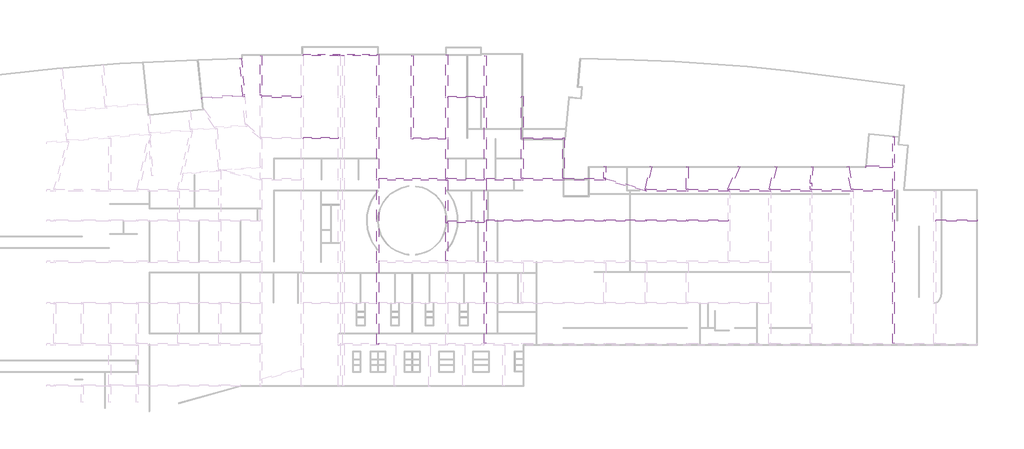
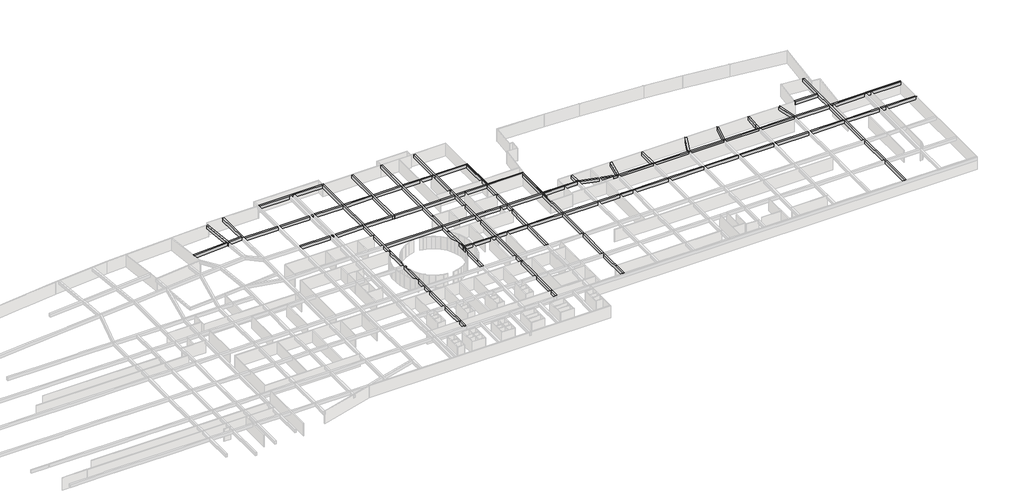
# One storey, part 8 of 8: 36 beams.
"""IFC4 building model written with IfcOpenShell, lengths in millimetres."""

from ifc_helpers import new_model, si_unit, frame, origin, place, context, project, spatial, polyline, outline, extrude, faceted_brep, element, save

model = new_model("IFC4")

# Units and contexts
model_context = context("Model", 3, world=origin())
ifc_project = project(units=[si_unit("LENGTHUNIT", "METRE", prefix="MILLI")], contexts=[model_context])

# Site, building, storey
site = spatial("IfcSite", under=ifc_project)
building = spatial("IfcBuilding", under=site)
storey = spatial("IfcBuildingStorey", under=building, Name="户型图", Elevation=0.0)

# Beams
placement = place(None, origin())
element("IfcBeam", 1, ObjectType="混凝土 - 矩形梁 : KL_beam", at=placement, inside=storey, context=model_context, shape_type="Brep", body=[
    faceted_brep([(535153.8653576, 24850.6327939, 3300.0), (535553.8653576, 24850.6327939, 3300.0), (535553.8653576, 24850.6327939, 2500.0), (535153.8653576, 24850.6327939, 2500.0), (535153.8653576, 18438.6264904, 3300.0), (535153.8653576, 18038.6264904, 3300.0), (535153.8653576, 13338.6264904, 3300.0), (535153.8653576, 12938.6264904, 3300.0), (535153.8653576, 6738.6264904, 3300.0), (535153.8653576, 6338.6264904, 3300.0), (535153.8653576, -2261.3735096, 3300.0), (535153.8653576, -2661.3735096, 3300.0), (535153.8653576, -11261.3735096, 3300.0), (535153.8653576, -11661.3735096, 3300.0), (535153.8653576, -20261.3735096, 3300.0), (535553.8653576, -20261.3735096, 3300.0), (535553.8653576, -11661.3735096, 3300.0), (535553.8653576, -11261.3735096, 3300.0), (535553.8653576, -2661.3735096, 3300.0), (535553.8653576, -2261.3735096, 3300.0), (535553.8653576, 6338.6264904, 3300.0), (535553.8653576, 6738.6264904, 3300.0), (535553.8653576, 12938.6264904, 3300.0), (535553.8653576, 13338.6264904, 3300.0), (535553.8653576, -20261.3735096, 2500.0), (535553.8653576, -11661.3735096, 2500.0), (535553.8653576, -11261.3735096, 2500.0), (535553.8653576, -2661.3735096, 2500.0), (535553.8653576, -2261.3735096, 2500.0), (535553.8653576, 6338.6264904, 2500.0), (535553.8653576, 6738.6264904, 2500.0), (535553.8653576, 12938.6264904, 2500.0), (535553.8653576, 13338.6264904, 2500.0), (535153.8653576, -20261.3735096, 2500.0), (535153.8653576, -11661.3735096, 2500.0), (535153.8653576, -11261.3735096, 2500.0), (535153.8653576, -2661.3735096, 2500.0), (535153.8653576, -2261.3735096, 2500.0), (535153.8653576, 6338.6264904, 2500.0), (535153.8653576, 6738.6264904, 2500.0), (535153.8653576, 12938.6264904, 2500.0), (535153.8653576, 13338.6264904, 2500.0), (535153.8653576, 18038.6264904, 2500.0), (535153.8653576, 18438.6264904, 2500.0)], [[[0, 1, 2, 3]], [[1, 0, 4, 5, 6, 7, 8, 9, 10, 11, 12, 13, 14, 15, 16, 17, 18, 19, 20, 21, 22, 23]], [[2, 1, 23, 22, 21, 20, 19, 18, 17, 16, 15, 24, 25, 26, 27, 28, 29, 30, 31, 32]], [[3, 2, 32, 31, 30, 29, 28, 27, 26, 25, 24, 33, 34, 35, 36, 37, 38, 39, 40, 41, 42, 43]], [[0, 3, 43, 42, 41, 40, 39, 38, 37, 36, 35, 34, 33, 14, 13, 12, 11, 10, 9, 8, 7, 6, 5, 4]], [[15, 14, 33, 24]]]),
])
element("IfcBeam", 2, ObjectType="混凝土 - 矩形梁 : KL_beam", at=placement, inside=storey, context=model_context, shape_type="SweptSolid", body=[
    extrude(outline(polyline([(553653.8653576, 6738.6264904), (553653.8653576, 6338.6264904), (544553.8653576, 6338.6264904), (544553.8653576, 6738.6264904), (553653.8653576, 6738.6264904)])), frame((0.0, 0.0, 2500.0), z_axis=(0.0, 0.0, 1.0), x_axis=(1.0, 0.0, 0.0)), (0.0, 0.0, 1.0), 800.0),
    extrude(outline(polyline([(544153.8653576, 6738.6264904), (544153.8653576, 6338.6264904), (535553.8653576, 6338.6264904), (535553.8653576, 6738.6264904), (544153.8653576, 6738.6264904)])), frame((0.0, 0.0, 2500.0), z_axis=(0.0, 0.0, 1.0), x_axis=(1.0, 0.0, 0.0)), (0.0, 0.0, 1.0), 800.0),
    extrude(outline(polyline([(535153.8653576, 6738.6264904), (535153.8653576, 6338.6264904), (526553.8653576, 6338.6264904), (526553.8653576, 6738.6264904), (535153.8653576, 6738.6264904)])), frame((0.0, 0.0, 2500.0), z_axis=(0.0, 0.0, 1.0), x_axis=(1.0, 0.0, 0.0)), (0.0, 0.0, 1.0), 800.0),
    extrude(outline(polyline([(526153.8653576, 6738.6264904), (526153.8653576, 6338.6264904), (517553.8653576, 6338.6264904), (517553.8653576, 6738.6264904), (526153.8653576, 6738.6264904)])), frame((0.0, 0.0, 2500.0), z_axis=(0.0, 0.0, 1.0), x_axis=(1.0, 0.0, 0.0)), (0.0, 0.0, 1.0), 800.0),
    extrude(outline(polyline([(517153.8653576, 6738.6264904), (517153.8653576, 6338.6264904), (508553.8653576, 6338.6264904), (508553.8653576, 6738.6264904), (517153.8653576, 6738.6264904)])), frame((0.0, 0.0, 2500.0), z_axis=(0.0, 0.0, 1.0), x_axis=(1.0, 0.0, 0.0)), (0.0, 0.0, 1.0), 800.0),
    extrude(outline(polyline([(508153.8653576, 6738.6264904), (508153.8653576, 6338.6264904), (499653.8653576, 6338.6264904), (499653.8653576, 6738.6264904), (508153.8653576, 6738.6264904)])), frame((0.0, 0.0, 2500.0), z_axis=(0.0, 0.0, 1.0), x_axis=(1.0, 0.0, 0.0)), (0.0, 0.0, 1.0), 800.0),
])
element("IfcBeam", 3, ObjectType="混凝土 - 矩形梁 : KL_beam", at=placement, inside=storey, context=model_context, shape_type="Brep", body=[
    faceted_brep([(553518.3052108, 13338.6264904, 3300.0), (553518.3052108, 12938.6264904, 3300.0), (553518.3052108, 12938.6264904, 2500.0), (553518.3052108, 13338.6264904, 2500.0), (535553.8653576, 13338.6264904, 3300.0), (535553.8653576, 12938.6264904, 3300.0), (544153.8653576, 12938.6264904, 3300.0), (544553.8653576, 12938.6264904, 3300.0), (535553.8653576, 12938.6264904, 2500.0), (544153.8653576, 12938.6264904, 2500.0), (544553.8653576, 12938.6264904, 2500.0), (535553.8653576, 13338.6264904, 2500.0)], [[[0, 1, 2, 3]], [[1, 0, 4, 5, 6, 7]], [[2, 1, 7, 6, 5, 8, 9, 10]], [[3, 2, 10, 9, 8, 11]], [[0, 3, 11, 4]], [[5, 4, 11, 8]]]),
    faceted_brep([(535153.8653576, 13338.6264904, 3300.0), (535153.8653576, 12938.6264904, 3300.0), (535153.8653576, 12938.6264904, 2500.0), (535153.8653576, 13338.6264904, 2500.0), (499253.8653576, 13338.6264904, 3300.0), (499253.8653576, 12938.6264904, 3300.0), (499653.8653576, 12938.6264904, 3300.0), (508153.8653576, 12938.6264904, 3300.0), (508553.8653576, 12938.6264904, 3300.0), (517153.8653576, 12938.6264904, 3300.0), (517553.8653576, 12938.6264904, 3300.0), (526153.8653576, 12938.6264904, 3300.0), (526553.8653576, 12938.6264904, 3300.0), (526518.7326348, 13338.6264904, 3300.0), (526111.2459568, 13338.6264904, 3300.0), (517553.8653576, 13338.6264904, 3300.0), (517153.8653576, 13338.6264904, 3300.0), (508609.8536841, 13338.6264904, 3300.0), (508197.6082323, 13338.6264904, 3300.0), (499656.0323963, 13338.6264904, 3300.0), (499253.8653576, 12938.6264904, 2500.0), (499653.8653576, 12938.6264904, 2500.0), (508153.8653576, 12938.6264904, 2500.0), (508553.8653576, 12938.6264904, 2500.0), (517153.8653576, 12938.6264904, 2500.0), (517553.8653576, 12938.6264904, 2500.0), (526153.8653576, 12938.6264904, 2500.0), (526553.8653576, 12938.6264904, 2500.0), (499253.8653576, 13338.6264904, 2500.0), (499656.0323963, 13338.6264904, 2500.0), (508197.6082323, 13338.6264904, 2500.0), (508609.8536841, 13338.6264904, 2500.0), (517153.8653576, 13338.6264904, 2500.0), (517553.8653576, 13338.6264904, 2500.0), (526111.2459568, 13338.6264904, 2500.0), (526518.7326348, 13338.6264904, 2500.0)], [[[0, 1, 2, 3]], [[4, 5, 6, 7, 8, 9, 10, 11, 12, 1, 0, 13, 14, 15, 16, 17, 18, 19]], [[5, 20, 21, 22, 23, 24, 25, 26, 27, 2, 1, 12, 11, 10, 9, 8, 7, 6]], [[20, 28, 29, 30, 31, 32, 33, 34, 35, 3, 2, 27, 26, 25, 24, 23, 22, 21]], [[28, 4, 19, 18, 17, 16, 15, 14, 13, 0, 3, 35, 34, 33, 32, 31, 30, 29]], [[5, 4, 28, 20]]]),
])
element("IfcBeam", 4, ObjectType="混凝土 - 矩形梁 : KL_beam", at=placement, inside=storey, context=model_context, shape_type="Brep", body=[
    faceted_brep([(499253.8653576, 6338.6264904, 3300.0), (499253.8653576, 6738.6264904, 3300.0), (490553.8653576, 6738.6264904, 3300.0), (490153.8653576, 6738.6264904, 3300.0), (481553.8653576, 6738.6264904, 3300.0), (481153.8653576, 6738.6264904, 3300.0), (472553.8653576, 6738.6264904, 3300.0), (472153.8653576, 6738.6264904, 3300.0), (463553.8653576, 6738.6264904, 3300.0), (463153.8653576, 6738.6264904, 3300.0), (454553.8653576, 6738.6264904, 3300.0), (454153.8653576, 6738.6264904, 3300.0), (446453.8653576, 6738.6264904, 3300.0), (446453.8653576, 6338.6264904, 3300.0), (454153.8653576, 6338.6264904, 3300.0), (454553.8653576, 6338.6264904, 3300.0), (463153.8653576, 6338.6264904, 3300.0), (463553.8653576, 6338.6264904, 3300.0), (472153.8653576, 6338.6264904, 3300.0), (472553.8653576, 6338.6264904, 3300.0), (481153.8653576, 6338.6264904, 3300.0), (481553.8653576, 6338.6264904, 3300.0), (490153.8653576, 6338.6264904, 3300.0), (490553.8653576, 6338.6264904, 3300.0), (499253.8653576, 6338.6264904, 2500.0), (446453.8653576, 6338.6264904, 2500.0), (454153.8653576, 6338.6264904, 2500.0), (454553.8653576, 6338.6264904, 2500.0), (463153.8653576, 6338.6264904, 2500.0), (463553.8653576, 6338.6264904, 2500.0), (472153.8653576, 6338.6264904, 2500.0), (472553.8653576, 6338.6264904, 2500.0), (481153.8653576, 6338.6264904, 2500.0), (481553.8653576, 6338.6264904, 2500.0), (490153.8653576, 6338.6264904, 2500.0), (490553.8653576, 6338.6264904, 2500.0), (499253.8653576, 6738.6264904, 2500.0), (446453.8653576, 6738.6264904, 2500.0), (454153.8653576, 6738.6264904, 2500.0), (454553.8653576, 6738.6264904, 2500.0), (463153.8653576, 6738.6264904, 2500.0), (463553.8653576, 6738.6264904, 2500.0), (472153.8653576, 6738.6264904, 2500.0), (472553.8653576, 6738.6264904, 2500.0), (481153.8653576, 6738.6264904, 2500.0), (481553.8653576, 6738.6264904, 2500.0), (490153.8653576, 6738.6264904, 2500.0), (490553.8653576, 6738.6264904, 2500.0)], [[[0, 1, 2, 3, 4, 5, 6, 7, 8, 9, 10, 11, 12, 13, 14, 15, 16, 17, 18, 19, 20, 21, 22, 23]], [[24, 0, 23, 22, 21, 20, 19, 18, 17, 16, 15, 14, 13, 25, 26, 27, 28, 29, 30, 31, 32, 33, 34, 35]], [[36, 24, 35, 34, 33, 32, 31, 30, 29, 28, 27, 26, 25, 37, 38, 39, 40, 41, 42, 43, 44, 45, 46, 47]], [[1, 36, 47, 46, 45, 44, 43, 42, 41, 40, 39, 38, 37, 12, 11, 10, 9, 8, 7, 6, 5, 4, 3, 2]], [[1, 0, 24, 36]], [[13, 12, 37, 25]]]),
])
element("IfcBeam", 5, ObjectType="混凝土 - 矩形梁 : KL_beam", at=placement, inside=storey, context=model_context, shape_type="Brep", body=[
    faceted_brep([(481153.8653576, 13338.6264904, 3300.0), (481153.8653576, 13157.8287437, 3300.0), (481153.8653576, 12984.9708278, 3300.0), (481153.8653576, 12938.6264904, 3300.0), (481553.8653576, 12938.6264904, 3300.0), (490153.8653576, 12938.6264904, 3300.0), (490553.8653576, 12938.6264904, 3300.0), (499253.8653576, 12938.6264904, 3300.0), (499253.8653576, 13338.6264904, 3300.0), (499221.4882454, 13338.6264904, 3300.0), (490553.8653576, 13338.6264904, 3300.0), (490153.8653576, 13338.6264904, 3300.0), (481596.3487482, 13338.6264904, 3300.0), (481188.9056055, 13338.6264904, 3300.0), (481153.8653576, 13338.6264904, 2500.0), (499253.8653576, 13338.6264904, 2500.0), (499221.4882454, 13338.6264904, 2500.0), (490553.8653576, 13338.6264904, 2500.0), (490153.8653576, 13338.6264904, 2500.0), (481596.3487482, 13338.6264904, 2500.0), (481188.9056055, 13338.6264904, 2500.0), (481153.8653576, 12938.6264904, 2500.0), (481153.8653576, 12984.9708278, 2500.0), (481153.8653576, 13157.8287437, 2500.0), (499253.8653576, 12938.6264904, 2500.0), (490553.8653576, 12938.6264904, 2500.0), (490153.8653576, 12938.6264904, 2500.0), (481553.8653576, 12938.6264904, 2500.0)], [[[0, 1, 2, 3, 4, 5, 6, 7, 8, 9, 10, 11, 12, 13]], [[14, 0, 13, 12, 11, 10, 9, 8, 15, 16, 17, 18, 19, 20]], [[21, 22, 23, 14, 20, 19, 18, 17, 16, 15, 24, 25, 26, 27]], [[3, 21, 27, 26, 25, 24, 7, 6, 5, 4]], [[3, 2, 1, 0, 14, 23, 22, 21]], [[8, 7, 24, 15]]]),
])
element("IfcBeam", 6, ObjectType="混凝土 - 矩形梁 : KL_beam", at=placement, inside=storey, context=model_context, shape_type="Brep", body=[
    faceted_brep([(472553.8653576, 15338.6264904, 3300.0), (472553.8653576, 15692.282153, 3300.0), (472553.8653576, 15738.6264904, 3300.0), (472380.0740924, 15738.6264904, 3300.0), (472153.8653576, 15738.6264904, 3300.0), (463553.8653576, 15738.6264904, 3300.0), (463153.8653576, 15738.6264904, 3300.0), (454553.8653576, 15738.6264904, 3300.0), (454153.8653576, 15738.6264904, 3300.0), (446453.8653576, 15738.6264904, 3300.0), (446453.8653576, 15338.6264904, 3300.0), (454153.8653576, 15338.6264904, 3300.0), (454553.8653576, 15338.6264904, 3300.0), (463153.8653576, 15338.6264904, 3300.0), (463553.8653576, 15338.6264904, 3300.0), (472153.8653576, 15338.6264904, 3300.0), (472553.8653576, 15738.6264904, 2500.0), (472380.0740924, 15738.6264904, 2500.0), (472153.8653576, 15738.6264904, 2500.0), (463553.8653576, 15738.6264904, 2500.0), (463153.8653576, 15738.6264904, 2500.0), (454553.8653576, 15738.6264904, 2500.0), (454153.8653576, 15738.6264904, 2500.0), (446453.8653576, 15738.6264904, 2500.0), (472553.8653576, 15692.282153, 2500.0), (472553.8653576, 15338.6264904, 2500.0), (472153.8653576, 15338.6264904, 2500.0), (463553.8653576, 15338.6264904, 2500.0), (463153.8653576, 15338.6264904, 2500.0), (454553.8653576, 15338.6264904, 2500.0), (454153.8653576, 15338.6264904, 2500.0), (446453.8653576, 15338.6264904, 2500.0)], [[[0, 1, 2, 3, 4, 5, 6, 7, 8, 9, 10, 11, 12, 13, 14, 15]], [[2, 16, 17, 18, 19, 20, 21, 22, 23, 9, 8, 7, 6, 5, 4, 3]], [[16, 24, 25, 26, 27, 28, 29, 30, 31, 23, 22, 21, 20, 19, 18, 17]], [[25, 0, 15, 14, 13, 12, 11, 10, 31, 30, 29, 28, 27, 26]], [[2, 1, 0, 25, 24, 16]], [[10, 9, 23, 31]]]),
])
element("IfcBeam", 7, ObjectType="混凝土 - 矩形梁 : KL_beam", at=placement, inside=storey, context=model_context, shape_type="Brep", body=[
    faceted_brep([(463153.8653576, -20261.3735096, 3300.0), (463553.8653576, -20261.3735096, 3300.0), (463553.8653576, -11661.3735096, 3300.0), (463153.8653576, -11661.3735096, 3300.0), (463553.8653576, -20261.3735096, 2500.0), (463553.8653576, -11661.3735096, 2500.0), (463153.8653576, -20261.3735096, 2500.0), (463153.8653576, -11661.3735096, 2500.0)], [[[0, 1, 2, 3]], [[1, 4, 5, 2]], [[4, 6, 7, 5]], [[6, 0, 3, 7]], [[1, 0, 6, 4]], [[3, 2, 5, 7]]]),
    faceted_brep([(463553.8653576, -2261.3735096, 3300.0), (463153.8653576, -2261.3735096, 3300.0), (463153.8653576, -2261.3735096, 2500.0), (463553.8653576, -2261.3735096, 2500.0), (463153.8653576, 6338.6264904, 3300.0), (463553.8653576, 6338.6264904, 3300.0), (463553.8653576, 6338.6264904, 2500.0), (463153.8653576, 6338.6264904, 2500.0)], [[[0, 1, 2, 3]], [[4, 5, 6, 7]], [[1, 0, 5, 4]], [[0, 3, 6, 5]], [[3, 2, 7, 6]], [[2, 1, 4, 7]]]),
    faceted_brep([(463153.8653576, -2661.3735096, 3300.0), (463553.8653576, -2661.3735096, 3300.0), (463553.8653576, -2661.3735096, 2500.0), (463153.8653576, -2661.3735096, 2500.0), (463553.8653576, -11261.3735096, 3300.0), (463153.8653576, -11261.3735096, 3300.0), (463153.8653576, -11261.3735096, 2500.0), (463553.8653576, -11261.3735096, 2500.0)], [[[0, 1, 2, 3]], [[4, 5, 6, 7]], [[1, 0, 5, 4]], [[2, 1, 4, 7]], [[3, 2, 7, 6]], [[0, 3, 6, 5]]]),
    faceted_brep([(463153.8653576, 6738.6264904, 3300.0), (463553.8653576, 6738.6264904, 3300.0), (463553.8653576, 15338.6264904, 3300.0), (463153.8653576, 15338.6264904, 3300.0), (463553.8653576, 6738.6264904, 2500.0), (463553.8653576, 15338.6264904, 2500.0), (463153.8653576, 6738.6264904, 2500.0), (463153.8653576, 15338.6264904, 2500.0)], [[[0, 1, 2, 3]], [[1, 4, 5, 2]], [[4, 6, 7, 5]], [[6, 0, 3, 7]], [[1, 0, 6, 4]], [[3, 2, 5, 7]]]),
    faceted_brep([(463553.8653576, 15738.6264904, 3300.0), (463153.8653576, 15738.6264904, 3300.0), (463153.8653576, 15738.6264904, 2500.0), (463553.8653576, 15738.6264904, 2500.0), (463153.8653576, 24638.6264904, 3300.0), (463553.8653576, 24638.6264904, 3300.0), (463553.8653576, 24638.6264904, 2500.0), (463153.8653576, 24638.6264904, 2500.0), (463153.8653576, 24238.6264904, 3300.0), (463153.8653576, 24238.6264904, 2500.0)], [[[0, 1, 2, 3]], [[4, 5, 6, 7]], [[5, 4, 8, 1, 0]], [[6, 5, 0, 3]], [[7, 6, 3, 2, 9]], [[4, 7, 9, 2, 1, 8]]]),
])
element("IfcBeam", 8, ObjectType="混凝土 - 矩形梁 : KL_beam", at=placement, inside=storey, context=model_context, shape_type="SweptSolid", body=[
    extrude(outline(polyline([(517153.8653576, 14643.8636747), (517553.8653576, 14633.3893061), (517553.8653576, 13338.6264904), (517153.8653576, 13338.6264904), (517153.8653576, 14643.8636747)])), frame((0.0, 0.0, 2500.0), z_axis=(0.0, 0.0, 1.0), x_axis=(1.0, 0.0, 0.0)), (0.0, 0.0, 1.0), 800.0),
])
element("IfcBeam", 9, ObjectType="混凝土 - 矩形梁 : KL_beam", at=placement, inside=storey, context=model_context, shape_type="SweptSolid", body=[
    extrude(outline(polyline([(517342.7828465, 18248.6241033), (517742.2346604, 18227.6897208), (517553.8653576, 14633.3893061), (517153.8653576, 14643.8636747), (517342.7828465, 18248.6241033)])), frame((0.0, 0.0, 2500.0), z_axis=(0.0, 0.0, 1.0), x_axis=(1.0, 0.0, 0.0)), (0.0, 0.0, 1.0), 800.0),
])
element("IfcBeam", 10, ObjectType="混凝土 - 矩形梁 : KL_beam", at=placement, inside=storey, context=model_context, shape_type="SweptSolid", body=[
    extrude(outline(polyline([(525146.7934929, 18300.3042867), (525539.4443663, 18376.6278849), (526518.7326348, 13338.6264904), (526111.2459568, 13338.6264904), (525146.7934929, 18300.3042867)])), frame((0.0, 0.0, 2500.0), z_axis=(0.0, 0.0, 1.0), x_axis=(1.0, 0.0, 0.0)), (0.0, 0.0, 1.0), 800.0),
])
element("IfcBeam", 11, ObjectType="混凝土 - 矩形梁 : KL_beam", at=placement, inside=storey, context=model_context, shape_type="SweptSolid", body=[
    extrude(outline(polyline([(529331.7779591, 18038.6264904), (529331.7779591, 18438.6264904), (535153.8653576, 18438.6264904), (535153.8653576, 18038.6264904), (529331.7779591, 18038.6264904)])), frame((0.0, 0.0, 2500.0), z_axis=(0.0, 0.0, 1.0), x_axis=(1.0, 0.0, 0.0)), (0.0, 0.0, 1.0), 800.0),
])
element("IfcBeam", 12, ObjectType="混凝土 - 矩形梁 : KL_beam", at=placement, inside=storey, context=model_context, shape_type="SweptSolid", body=[
    extrude(outline(polyline([(509441.992259, 18329.5782188), (509830.1105496, 18232.8094606), (508609.8536841, 13338.6264904), (508197.6082323, 13338.6264904), (509441.992259, 18329.5782188)])), frame((0.0, 0.0, 2500.0), z_axis=(0.0, 0.0, 1.0), x_axis=(1.0, 0.0, 0.0)), (0.0, 0.0, 1.0), 800.0),
])
element("IfcBeam", 13, ObjectType="混凝土 - 矩形梁 : KL_beam", at=placement, inside=storey, context=model_context, shape_type="Brep", body=[
    faceted_brep([(501377.0189815, 18416.7386747, 3300.0), (501745.2209229, 18260.4462233, 3300.0), (501745.2209229, 18260.4462233, 2500.0), (501377.0189815, 18416.7386747, 2500.0), (499221.4882454, 13338.6264904, 3300.0), (499253.8653576, 13338.6264904, 3300.0), (499656.0323963, 13338.6264904, 3300.0), (499656.0323963, 13338.6264904, 2500.0), (499253.8653576, 13338.6264904, 2500.0), (499221.4882454, 13338.6264904, 2500.0)], [[[0, 1, 2, 3]], [[1, 0, 4, 5, 6]], [[2, 1, 6, 7]], [[3, 2, 7, 8, 9]], [[0, 3, 9, 4]], [[4, 9, 8, 7, 6, 5]]]),
])
element("IfcBeam", 14, ObjectType="混凝土 - 矩形梁 : KL_beam", at=placement, inside=storey, context=model_context, shape_type="SweptSolid", body=[
    extrude(outline(polyline([(490153.8653576, 18238.6264904), (490553.8653576, 18238.6264904), (490553.8653576, 13338.6264904), (490153.8653576, 13338.6264904), (490153.8653576, 18238.6264904)])), frame((0.0, 0.0, 2500.0), z_axis=(0.0, 0.0, 1.0), x_axis=(1.0, 0.0, 0.0)), (0.0, 0.0, 1.0), 800.0),
])
element("IfcBeam", 15, ObjectType="混凝土 - 矩形梁 : KL_beam", at=placement, inside=storey, context=model_context, shape_type="Brep", body=[
    faceted_brep([(482165.253861, 18376.3067336, 3300.0), (482557.9466891, 18300.1992914, 3300.0), (482557.9466891, 18300.1992914, 2500.0), (482165.253861, 18376.3067336, 2500.0), (481198.3001251, 13387.0995484, 3300.0), (481188.9056055, 13338.6264904, 3300.0), (481553.8653576, 13338.6264904, 3300.0), (481596.3487482, 13338.6264904, 3300.0), (481596.3487482, 13338.6264904, 2500.0), (481553.8653576, 13338.6264904, 2500.0), (481188.9056055, 13338.6264904, 2500.0), (481198.3001251, 13387.0995484, 2500.0)], [[[0, 1, 2, 3]], [[1, 0, 4, 5, 6, 7]], [[2, 1, 7, 8]], [[3, 2, 8, 9, 10, 11]], [[0, 3, 11, 10, 5, 4]], [[8, 7, 6, 5, 10, 9]]]),
    faceted_brep([(481153.8653576, 13157.8287437, 3300.0), (481153.8653576, 12984.9708278, 3300.0), (481153.8653576, 12984.9708278, 2500.0), (481153.8653576, 13157.8287437, 2500.0), (481122.0102694, 12993.465518, 3300.0), (481122.0102694, 12993.465518, 2500.0)], [[[0, 1, 2, 3]], [[4, 5, 2, 1]], [[1, 0, 4]], [[3, 2, 5]], [[0, 3, 5, 4]]]),
])
element("IfcBeam", 16, ObjectType="混凝土 - 矩形梁 : KL_beam", at=placement, inside=storey, context=model_context, shape_type="Brep", body=[
    faceted_brep([(481198.3001251, 13387.0995484, 3300.0), (481198.3001251, 13387.0995484, 2500.0), (472553.8653576, 15692.282153, 2500.0), (472553.8653576, 15692.282153, 3300.0), (481153.8653576, 13338.6264904, 3300.0), (481153.8653576, 13338.6264904, 2500.0), (481188.9056055, 13338.6264904, 2500.0), (481188.9056055, 13338.6264904, 3300.0), (481153.8653576, 13157.8287437, 3300.0), (481153.8653576, 13157.8287437, 2500.0), (472553.8653576, 15338.6264904, 3300.0), (472553.8653576, 15278.3041611, 3300.0), (481122.0102694, 12993.465518, 3300.0), (481122.0102694, 12993.465518, 2500.0), (472553.8653576, 15278.3041611, 2500.0), (472553.8653576, 15338.6264904, 2500.0)], [[[0, 1, 2, 3]], [[4, 5, 6, 7]], [[5, 4, 8, 9]], [[8, 4, 7, 0, 3, 10, 11, 12]], [[13, 12, 11, 14]], [[6, 5, 9, 13, 14, 15, 2, 1]], [[1, 0, 7, 6]], [[9, 8, 12, 13]], [[3, 2, 15, 14, 11, 10]]]),
    faceted_brep([(472153.8653576, 15738.6264904, 2500.0), (472153.8653576, 15738.6264904, 3300.0), (472153.8653576, 15798.9488197, 3300.0), (472153.8653576, 15798.9488197, 2500.0), (472380.0740924, 15738.6264904, 2500.0), (472380.0740924, 15738.6264904, 3300.0)], [[[0, 1, 2, 3]], [[4, 5, 1, 0]], [[4, 3, 2, 5]], [[5, 2, 1]], [[3, 4, 0]]]),
])
element("IfcBeam", 17, ObjectType="混凝土 - 矩形梁 : KL_beam", at=placement, inside=storey, context=model_context, shape_type="SweptSolid", body=[
    extrude(outline(polyline([(472153.8653576, 18338.6264904), (472553.8653576, 18338.6264904), (472553.8653576, 15738.6264904), (472380.0740924, 15738.6264904), (472153.8653576, 15798.9488197), (472153.8653576, 18338.6264904)])), frame((0.0, 0.0, 2500.0), z_axis=(0.0, 0.0, 1.0), x_axis=(1.0, 0.0, 0.0)), (0.0, 0.0, 1.0), 800.0),
])
element("IfcBeam", 18, ObjectType="混凝土 - 矩形梁 : KL_beam", at=placement, inside=storey, context=model_context, shape_type="Brep", body=[
    faceted_brep([(454153.8653576, -2261.3735096, 3300.0), (454553.8653576, -2261.3735096, 3300.0), (454553.8653576, 6338.6264904, 3300.0), (454153.8653576, 6338.6264904, 3300.0), (454553.8653576, -2261.3735096, 2500.0), (454553.8653576, 6338.6264904, 2500.0), (454153.8653576, -2261.3735096, 2500.0), (454153.8653576, 6338.6264904, 2500.0)], [[[0, 1, 2, 3]], [[1, 4, 5, 2]], [[4, 6, 7, 5]], [[6, 0, 3, 7]], [[1, 0, 6, 4]], [[3, 2, 5, 7]]]),
    faceted_brep([(454553.8653576, 6738.6264904, 3300.0), (454153.8653576, 6738.6264904, 3300.0), (454153.8653576, 6738.6264904, 2500.0), (454553.8653576, 6738.6264904, 2500.0), (454153.8653576, 15338.6264904, 3300.0), (454553.8653576, 15338.6264904, 3300.0), (454553.8653576, 15338.6264904, 2500.0), (454153.8653576, 15338.6264904, 2500.0)], [[[0, 1, 2, 3]], [[4, 5, 6, 7]], [[1, 0, 5, 4]], [[0, 3, 6, 5]], [[3, 2, 7, 6]], [[2, 1, 4, 7]]]),
    faceted_brep([(454553.8653576, 33688.6264755, 3300.0), (454153.8653576, 33688.6264755, 3300.0), (454153.8653576, 33288.6264755, 3300.0), (454153.8653576, 24638.6264904, 3300.0), (454153.8653576, 24238.6264904, 3300.0), (454153.8653576, 15738.6264904, 3300.0), (454553.8653576, 15738.6264904, 3300.0), (454553.8653576, 24238.6264904, 3300.0), (454553.8653576, 24638.6264904, 3300.0), (454553.8653576, 33688.6264755, 2500.0), (454553.8653576, 15738.6264904, 2500.0), (454553.8653576, 24238.6264904, 2500.0), (454553.8653576, 24638.6264904, 2500.0), (454153.8653576, 33688.6264755, 2500.0), (454153.8653576, 15738.6264904, 2500.0), (454153.8653576, 24238.6264904, 2500.0), (454153.8653576, 24638.6264904, 2500.0), (454153.8653576, 33288.6264755, 2500.0)], [[[0, 1, 2, 3, 4, 5, 6, 7, 8]], [[9, 0, 8, 7, 6, 10, 11, 12]], [[13, 9, 12, 11, 10, 14, 15, 16, 17]], [[1, 13, 17, 16, 15, 14, 5, 4, 3, 2]], [[6, 5, 14, 10]], [[1, 0, 9, 13]]]),
])
element("IfcBeam", 19, ObjectType="混凝土 - 矩形梁 : KL_beam", at=placement, inside=storey, context=model_context, shape_type="Brep", body=[
    faceted_brep([(446453.8653576, 42538.6264904, 3300.0), (446453.8653576, 42538.6264904, 2500.0), (446053.8653576, 42538.6264904, 2500.0), (446053.8653576, 42538.6264904, 3300.0), (446053.8653576, 33688.6264755, 3300.0), (446053.8653576, 33288.6264755, 3300.0), (446053.8653576, 24638.6264904, 3300.0), (446053.8653576, 24238.6264904, 3300.0), (446053.8653576, 15738.6264904, 3300.0), (446053.8653576, 15338.6264904, 3300.0), (446053.8653576, 6488.6264674, 3300.0), (446053.8653576, 6088.6264674, 3300.0), (446053.8653576, -2261.3735096, 3300.0), (446053.8653576, -2661.3735096, 3300.0), (446053.8653576, -11261.3735096, 3300.0), (446053.8653576, -11661.3735096, 3300.0), (446053.8653576, -20261.3735096, 3300.0), (446453.8653576, -20261.3735096, 3300.0), (446453.8653576, -11661.3735096, 3300.0), (446453.8653576, -11261.3735096, 3300.0), (446453.8653576, -2661.3735096, 3300.0), (446453.8653576, -2261.3735096, 3300.0), (446453.8653576, 6338.6264904, 3300.0), (446453.8653576, 6738.6264904, 3300.0), (446453.8653576, 15338.6264904, 3300.0), (446453.8653576, 15738.6264904, 3300.0), (446453.8653576, 24238.6264904, 3300.0), (446453.8653576, 24638.6264904, 3300.0), (446453.8653576, 33288.6264755, 3300.0), (446453.8653576, 33688.6264755, 3300.0), (446053.8653576, 33688.6264755, 2500.0), (446053.8653576, 33288.6264755, 2500.0), (446053.8653576, 24638.6264904, 2500.0), (446053.8653576, 24238.6264904, 2500.0), (446053.8653576, 15738.6264904, 2500.0), (446053.8653576, 15338.6264904, 2500.0), (446053.8653576, 6488.6264674, 2500.0), (446053.8653576, 6088.6264674, 2500.0), (446053.8653576, -2261.3735096, 2500.0), (446053.8653576, -2661.3735096, 2500.0), (446053.8653576, -11261.3735096, 2500.0), (446053.8653576, -11661.3735096, 2500.0), (446053.8653576, -20261.3735096, 2500.0), (446453.8653576, 33688.6264755, 2500.0), (446453.8653576, 33288.6264755, 2500.0), (446453.8653576, 24638.6264904, 2500.0), (446453.8653576, 24238.6264904, 2500.0), (446453.8653576, 15738.6264904, 2500.0), (446453.8653576, 15338.6264904, 2500.0), (446453.8653576, 6738.6264904, 2500.0), (446453.8653576, 6338.6264904, 2500.0), (446453.8653576, -2261.3735096, 2500.0), (446453.8653576, -2661.3735096, 2500.0), (446453.8653576, -11261.3735096, 2500.0), (446453.8653576, -11661.3735096, 2500.0), (446453.8653576, -20261.3735096, 2500.0)], [[[0, 1, 2, 3]], [[0, 3, 4, 5, 6, 7, 8, 9, 10, 11, 12, 13, 14, 15, 16, 17, 18, 19, 20, 21, 22, 23, 24, 25, 26, 27, 28, 29]], [[3, 2, 30, 31, 32, 33, 34, 35, 36, 37, 38, 39, 40, 41, 42, 16, 15, 14, 13, 12, 11, 10, 9, 8, 7, 6, 5, 4]], [[2, 1, 43, 44, 45, 46, 47, 48, 49, 50, 51, 52, 53, 54, 55, 42, 41, 40, 39, 38, 37, 36, 35, 34, 33, 32, 31, 30]], [[1, 0, 29, 28, 27, 26, 25, 24, 23, 22, 21, 20, 19, 18, 17, 55, 54, 53, 52, 51, 50, 49, 48, 47, 46, 45, 44, 43]], [[17, 16, 42, 55]]]),
])
element("IfcBeam", 20, ObjectType="混凝土 - 矩形梁 : KL_beam", at=placement, inside=storey, context=model_context, shape_type="Brep", body=[
    faceted_brep([(437653.8653576, 15738.6264904, 3300.0), (437653.8653576, 15338.6264904, 3300.0), (438053.8653576, 15338.6264904, 3300.0), (446053.8653576, 15338.6264904, 3300.0), (446053.8653576, 15738.6264904, 3300.0), (438053.8653576, 15738.6264904, 3300.0), (437653.8653576, 15738.6264904, 2500.0), (446053.8653576, 15738.6264904, 2500.0), (438053.8653576, 15738.6264904, 2500.0), (437653.8653576, 15338.6264904, 2500.0), (446053.8653576, 15338.6264904, 2500.0), (438053.8653576, 15338.6264904, 2500.0)], [[[0, 1, 2, 3, 4, 5]], [[6, 0, 5, 4, 7, 8]], [[9, 6, 8, 7, 10, 11]], [[1, 9, 11, 10, 3, 2]], [[4, 3, 10, 7]], [[1, 0, 6, 9]]]),
])
element("IfcBeam", 21, ObjectType="混凝土 - 矩形梁 : KL_beam", at=placement, inside=storey, context=model_context, shape_type="Brep", body=[
    faceted_brep([(437653.8653576, 42735.0986184, 3300.0), (438053.8653576, 42735.0986184, 3300.0), (438053.8653576, 42735.0986184, 2500.0), (437653.8653576, 42735.0986184, 2500.0), (437653.8653576, 33688.6264755, 3300.0), (437653.8653576, 33288.6264755, 3300.0), (437653.8653576, 24638.6264904, 3300.0), (437653.8653576, 24238.6264904, 3300.0), (437653.8653576, 15738.6264904, 3300.0), (438053.8653576, 15738.6264904, 3300.0), (438053.8653576, 24238.6264904, 3300.0), (438053.8653576, 24638.6264904, 3300.0), (438053.8653576, 33288.6264755, 3300.0), (438053.8653576, 33688.6264755, 3300.0), (438053.8653576, 15738.6264904, 2500.0), (438053.8653576, 24238.6264904, 2500.0), (438053.8653576, 24638.6264904, 2500.0), (438053.8653576, 33288.6264755, 2500.0), (438053.8653576, 33688.6264755, 2500.0), (437653.8653576, 15738.6264904, 2500.0), (437653.8653576, 24238.6264904, 2500.0), (437653.8653576, 24638.6264904, 2500.0), (437653.8653576, 33288.6264755, 2500.0), (437653.8653576, 33688.6264755, 2500.0)], [[[0, 1, 2, 3]], [[1, 0, 4, 5, 6, 7, 8, 9, 10, 11, 12, 13]], [[2, 1, 13, 12, 11, 10, 9, 14, 15, 16, 17, 18]], [[3, 2, 18, 17, 16, 15, 14, 19, 20, 21, 22, 23]], [[0, 3, 23, 22, 21, 20, 19, 8, 7, 6, 5, 4]], [[9, 8, 19, 14]]]),
])
element("IfcBeam", 22, ObjectType="混凝土 - 矩形梁 : KL_beam", at=placement, inside=storey, context=model_context, shape_type="Brep", body=[
    faceted_brep([(430553.8653642, 42538.6264755, 3300.0), (430553.8653642, 42538.6264755, 2500.0), (430153.8653642, 42538.6264755, 2500.0), (430153.8653642, 42538.6264755, 3300.0), (430153.8653642, 33738.6264904, 3300.0), (430153.8653642, 33338.6264904, 3300.0), (430153.8653642, 24738.6264659, 3300.0), (430153.8653642, 24338.6264659, 3300.0), (430153.8653642, 24238.6264904, 3300.0), (430553.8653642, 24238.6264904, 3300.0), (430553.8653642, 24638.6264904, 3300.0), (430553.8653642, 33288.6264755, 3300.0), (430553.8653642, 33688.6264755, 3300.0), (430153.8653642, 33738.6264904, 2500.0), (430153.8653642, 33338.6264904, 2500.0), (430153.8653642, 24738.6264659, 2500.0), (430153.8653642, 24338.6264659, 2500.0), (430153.8653642, 24238.6264904, 2500.0), (430553.8653642, 33688.6264755, 2500.0), (430553.8653642, 33288.6264755, 2500.0), (430553.8653642, 24638.6264904, 2500.0), (430553.8653642, 24238.6264904, 2500.0)], [[[0, 1, 2, 3]], [[0, 3, 4, 5, 6, 7, 8, 9, 10, 11, 12]], [[3, 2, 13, 14, 15, 16, 17, 8, 7, 6, 5, 4]], [[2, 1, 18, 19, 20, 21, 17, 16, 15, 14, 13]], [[1, 0, 12, 11, 10, 9, 21, 20, 19, 18]], [[9, 8, 17, 21]]]),
])
element("IfcBeam", 23, ObjectType="混凝土 - 矩形梁 : KL_beam", at=placement, inside=storey, context=model_context, shape_type="SweptSolid", body=[
    extrude(outline(polyline([(430553.8653642, 24238.6264904), (430553.8653642, 24638.6264904), (437653.8653576, 24638.6264904), (437653.8653576, 24238.6264904), (430553.8653642, 24238.6264904)])), frame((0.0, 0.0, 2500.0), z_axis=(0.0, 0.0, 1.0), x_axis=(1.0, 0.0, 0.0)), (0.0, 0.0, 1.0), 800.0),
])
element("IfcBeam", 24, ObjectType="混凝土 - 矩形梁 : KL_beam", at=placement, inside=storey, context=model_context, shape_type="SweptSolid", body=[
    extrude(outline(polyline([(438053.8653576, 24238.6264904), (438053.8653576, 24638.6264904), (446053.8653576, 24638.6264904), (446053.8653576, 24238.6264904), (438053.8653576, 24238.6264904)])), frame((0.0, 0.0, 2500.0), z_axis=(0.0, 0.0, 1.0), x_axis=(1.0, 0.0, 0.0)), (0.0, 0.0, 1.0), 800.0),
    extrude(outline(polyline([(463153.8653576, 24638.6264904), (463153.8653576, 24238.6264904), (454553.8653576, 24238.6264904), (454553.8653576, 24638.6264904), (463153.8653576, 24638.6264904)])), frame((0.0, 0.0, 2500.0), z_axis=(0.0, 0.0, 1.0), x_axis=(1.0, 0.0, 0.0)), (0.0, 0.0, 1.0), 800.0),
    extrude(outline(polyline([(454153.8653576, 24638.6264904), (454153.8653576, 24238.6264904), (446453.8653576, 24238.6264904), (446453.8653576, 24638.6264904), (454153.8653576, 24638.6264904)])), frame((0.0, 0.0, 2500.0), z_axis=(0.0, 0.0, 1.0), x_axis=(1.0, 0.0, 0.0)), (0.0, 0.0, 1.0), 800.0),
])
element("IfcBeam", 25, ObjectType="混凝土 - 矩形梁 : KL_beam", at=placement, inside=storey, context=model_context, shape_type="SweptSolid", body=[
    extrude(outline(polyline([(430553.8653642, 33288.6264755), (430553.8653642, 33688.6264755), (437653.8653576, 33688.6264755), (437653.8653576, 33288.6264755), (430553.8653642, 33288.6264755)])), frame((0.0, 0.0, 2500.0), z_axis=(0.0, 0.0, 1.0), x_axis=(1.0, 0.0, 0.0)), (0.0, 0.0, 1.0), 800.0),
    extrude(outline(polyline([(454153.8653576, 33688.6264755), (454153.8653576, 33288.6264755), (446453.8653576, 33288.6264755), (446453.8653576, 33688.6264755), (454153.8653576, 33688.6264755)])), frame((0.0, 0.0, 2500.0), z_axis=(0.0, 0.0, 1.0), x_axis=(1.0, 0.0, 0.0)), (0.0, 0.0, 1.0), 800.0),
    extrude(outline(polyline([(446053.8653576, 33688.6264755), (446053.8653576, 33288.6264755), (438053.8653576, 33288.6264755), (438053.8653576, 33688.6264755), (446053.8653576, 33688.6264755)])), frame((0.0, 0.0, 2500.0), z_axis=(0.0, 0.0, 1.0), x_axis=(1.0, 0.0, 0.0)), (0.0, 0.0, 1.0), 800.0),
])
element("IfcBeam", 26, ObjectType="混凝土 - 矩形梁 : KL_beam", at=placement, inside=storey, context=model_context, shape_type="Brep", body=[
    faceted_brep([(423053.8653576, -20460.9013816, 3300.0), (422653.8653576, -20460.9013816, 3300.0), (422653.8653576, -20460.9013816, 2500.0), (423053.8653576, -20460.9013816, 2500.0), (423053.8653576, -20261.3735096, 3300.0), (423053.8653576, -11661.3735096, 3300.0), (423053.8653576, -11261.3735096, 3300.0), (423053.8653576, -2661.3735096, 3300.0), (423053.8653576, -2261.3735096, 3300.0), (423053.8653576, 15338.6264904, 3300.0), (423053.8653576, 15738.6264904, 3300.0), (423053.8653576, 24338.6264659, 3300.0), (423053.8653576, 24738.6264659, 3300.0), (423053.8653576, 33338.6264904, 3300.0), (423053.8653576, 33738.6264904, 3300.0), (423053.8653576, 42835.5707464, 3300.0), (422653.8653576, 42835.5707464, 3300.0), (422653.8653576, 42435.5707464, 3300.0), (422653.8653576, 33738.6264904, 3300.0), (422653.8653576, 33338.6264904, 3300.0), (422653.8653576, 24738.6264659, 3300.0), (422653.8653576, 24338.6264659, 3300.0), (422653.8653576, 15738.6264904, 3300.0), (422653.8653576, 15338.6264904, 3300.0), (422653.8653576, 6738.6264904, 3300.0), (422653.8653576, 6338.6264904, 3300.0), (422653.8653576, -2261.3735096, 3300.0), (422653.8653576, -2661.3735096, 3300.0), (422653.8653576, -11261.3735096, 3300.0), (422653.8653576, -11661.3735096, 3300.0), (422653.8653576, -20261.3735096, 3300.0), (422653.8653576, 42835.5707464, 2500.0), (422653.8653576, 42435.5707464, 2500.0), (422653.8653576, 33738.6264904, 2500.0), (422653.8653576, 33338.6264904, 2500.0), (422653.8653576, 24738.6264659, 2500.0), (422653.8653576, 24338.6264659, 2500.0), (422653.8653576, 15738.6264904, 2500.0), (422653.8653576, 15338.6264904, 2500.0), (422653.8653576, 6738.6264904, 2500.0), (422653.8653576, 6338.6264904, 2500.0), (422653.8653576, -2261.3735096, 2500.0), (422653.8653576, -2661.3735096, 2500.0), (422653.8653576, -11261.3735096, 2500.0), (422653.8653576, -11661.3735096, 2500.0), (422653.8653576, -20261.3735096, 2500.0), (423053.8653576, 42835.5707464, 2500.0), (423053.8653576, 33738.6264904, 2500.0), (423053.8653576, 33338.6264904, 2500.0), (423053.8653576, 24738.6264659, 2500.0), (423053.8653576, 24338.6264659, 2500.0), (423053.8653576, 15738.6264904, 2500.0), (423053.8653576, 15338.6264904, 2500.0), (423053.8653576, -2261.3735096, 2500.0), (423053.8653576, -2661.3735096, 2500.0), (423053.8653576, -11261.3735096, 2500.0), (423053.8653576, -11661.3735096, 2500.0), (423053.8653576, -20261.3735096, 2500.0)], [[[0, 1, 2, 3]], [[1, 0, 4, 5, 6, 7, 8, 9, 10, 11, 12, 13, 14, 15, 16, 17, 18, 19, 20, 21, 22, 23, 24, 25, 26, 27, 28, 29, 30]], [[2, 1, 30, 29, 28, 27, 26, 25, 24, 23, 22, 21, 20, 19, 18, 17, 16, 31, 32, 33, 34, 35, 36, 37, 38, 39, 40, 41, 42, 43, 44, 45]], [[3, 2, 45, 44, 43, 42, 41, 40, 39, 38, 37, 36, 35, 34, 33, 32, 31, 46, 47, 48, 49, 50, 51, 52, 53, 54, 55, 56, 57]], [[0, 3, 57, 56, 55, 54, 53, 52, 51, 50, 49, 48, 47, 46, 15, 14, 13, 12, 11, 10, 9, 8, 7, 6, 5, 4]], [[16, 15, 46, 31]]]),
])
element("IfcBeam", 27, ObjectType="混凝土 - 矩形梁 : KL_beam", at=placement, inside=storey, context=model_context, shape_type="SweptSolid", body=[
    extrude(outline(polyline([(406153.8653576, 33738.6264904), (406153.8653576, 33338.6264904), (397553.8653576, 33338.6264904), (397553.8653576, 33738.6264904), (406153.8653576, 33738.6264904)])), frame((0.0, 0.0, 2500.0), z_axis=(0.0, 0.0, 1.0), x_axis=(1.0, 0.0, 0.0)), (0.0, 0.0, 1.0), 800.0),
    extrude(outline(polyline([(430153.8653642, 33738.6264904), (430153.8653642, 33338.6264904), (423053.8653576, 33338.6264904), (423053.8653576, 33738.6264904), (430153.8653642, 33738.6264904)])), frame((0.0, 0.0, 2500.0), z_axis=(0.0, 0.0, 1.0), x_axis=(1.0, 0.0, 0.0)), (0.0, 0.0, 1.0), 800.0),
    extrude(outline(polyline([(422653.8653576, 33738.6264904), (422653.8653576, 33338.6264904), (415553.8653576, 33338.6264904), (415553.8653576, 33738.6264904), (422653.8653576, 33738.6264904)])), frame((0.0, 0.0, 2500.0), z_axis=(0.0, 0.0, 1.0), x_axis=(1.0, 0.0, 0.0)), (0.0, 0.0, 1.0), 800.0),
    extrude(outline(polyline([(415153.8653576, 33738.6264904), (415153.8653576, 33338.6264904), (414653.8653576, 33338.6264904), (414653.8653576, 33738.6264904), (415153.8653576, 33738.6264904)])), frame((0.0, 0.0, 2500.0), z_axis=(0.0, 0.0, 1.0), x_axis=(1.0, 0.0, 0.0)), (0.0, 0.0, 1.0), 800.0),
    extrude(outline(polyline([(414253.8653576, 33738.6264904), (414253.8653576, 33338.6264904), (406553.8653576, 33338.6264904), (406553.8653576, 33738.6264904), (414253.8653576, 33738.6264904)])), frame((0.0, 0.0, 2500.0), z_axis=(0.0, 0.0, 1.0), x_axis=(1.0, 0.0, 0.0)), (0.0, 0.0, 1.0), 800.0),
])
element("IfcBeam", 28, ObjectType="混凝土 - 矩形梁 : KL_beam", at=placement, inside=storey, context=model_context, shape_type="Brep", body=[
    faceted_brep([(422653.8653576, 42435.5707464, 3300.0), (422653.8653576, 42835.5707464, 3300.0), (406553.8653576, 42835.5707464, 3300.0), (406553.8653576, 42435.5707464, 3300.0), (414253.8653576, 42435.5707464, 3300.0), (414653.8653576, 42435.5707464, 3300.0), (415153.8653576, 42435.5707464, 3300.0), (415553.8653576, 42435.5707464, 3300.0), (422653.8653576, 42435.5707464, 2500.0), (406553.8653576, 42435.5707464, 2500.0), (414253.8653576, 42435.5707464, 2500.0), (414653.8653576, 42435.5707464, 2500.0), (415153.8653576, 42435.5707464, 2500.0), (415553.8653576, 42435.5707464, 2500.0), (422653.8653576, 42835.5707464, 2500.0), (406553.8653576, 42835.5707464, 2500.0)], [[[0, 1, 2, 3, 4, 5, 6, 7]], [[8, 0, 7, 6, 5, 4, 3, 9, 10, 11, 12, 13]], [[14, 8, 13, 12, 11, 10, 9, 15]], [[1, 14, 15, 2]], [[1, 0, 8, 14]], [[3, 2, 15, 9]]]),
])
element("IfcBeam", 29, ObjectType="混凝土 - 矩形梁 : KL_beam", at=placement, inside=storey, context=model_context, shape_type="SweptSolid", body=[
    extrude(outline(polyline([(406553.8653576, 24338.6264659), (406553.8653576, 24738.6264659), (414253.8653576, 24738.6264659), (414253.8653576, 24338.6264659), (406553.8653576, 24338.6264659)])), frame((0.0, 0.0, 2500.0), z_axis=(0.0, 0.0, 1.0), x_axis=(1.0, 0.0, 0.0)), (0.0, 0.0, 1.0), 800.0),
    extrude(outline(polyline([(430153.8653642, 24738.6264659), (430153.8653642, 24338.6264659), (423053.8653576, 24338.6264659), (423053.8653576, 24738.6264659), (430153.8653642, 24738.6264659)])), frame((0.0, 0.0, 2500.0), z_axis=(0.0, 0.0, 1.0), x_axis=(1.0, 0.0, 0.0)), (0.0, 0.0, 1.0), 800.0),
    extrude(outline(polyline([(422653.8653576, 24738.6264659), (422653.8653576, 24338.6264659), (415553.8653576, 24338.6264659), (415553.8653576, 24738.6264659), (422653.8653576, 24738.6264659)])), frame((0.0, 0.0, 2500.0), z_axis=(0.0, 0.0, 1.0), x_axis=(1.0, 0.0, 0.0)), (0.0, 0.0, 1.0), 800.0),
    extrude(outline(polyline([(415153.8653576, 24738.6264659), (415153.8653576, 24338.6264659), (414653.8653576, 24338.6264659), (414653.8653576, 24738.6264659), (415153.8653576, 24738.6264659)])), frame((0.0, 0.0, 2500.0), z_axis=(0.0, 0.0, 1.0), x_axis=(1.0, 0.0, 0.0)), (0.0, 0.0, 1.0), 800.0),
])
element("IfcBeam", 30, ObjectType="混凝土 - 矩形梁 : KL_beam", at=placement, inside=storey, context=model_context, shape_type="Brep", body=[
    faceted_brep([(393079.365782, 41941.3589155, 3300.0), (393079.365782, 41941.3589155, 2500.0), (392680.7488852, 41908.12385, 2500.0), (392680.7488852, 41908.12385, 3300.0), (393379.9831682, 33521.6020788, 3300.0), (393778.5322172, 33555.650902, 3300.0), (393767.5509635, 33687.3585786, 3300.0), (393734.3129272, 34086.0111079, 3300.0), (393335.251638, 34058.1060242, 3300.0), (393368.4896744, 33659.4534949, 3300.0), (393379.9831682, 33521.6020788, 2500.0), (393335.251638, 34058.1060242, 2500.0), (393368.4896744, 33659.4534949, 2500.0), (393778.5322172, 33555.650902, 2500.0), (393734.3129272, 34086.0111079, 2500.0), (393767.5509635, 33687.3585786, 2500.0)], [[[0, 1, 2, 3]], [[4, 5, 6, 7, 0, 3, 8, 9]], [[10, 4, 9, 8, 3, 2, 11, 12]], [[13, 10, 12, 11, 2, 1, 14, 15]], [[5, 13, 15, 14, 1, 0, 7, 6]], [[5, 4, 10, 13]]]),
])
element("IfcBeam", 31, ObjectType="混凝土 - 矩形梁 : KL_beam", at=placement, inside=storey, context=model_context, shape_type="SweptSolid", body=[
    extrude(outline(polyline([(384450.262452, 33035.830297), (384422.3598625, 33434.8559171), (393335.251638, 34058.1060242), (393368.4896744, 33659.4534949), (384450.262452, 33035.830297)])), frame((0.0, 0.0, 2500.0), z_axis=(0.0, 0.0, 1.0), x_axis=(1.0, 0.0, 0.0)), (0.0, 0.0, 1.0), 800.0),
    extrude(outline(polyline([(393767.5509635, 33687.3585786), (393734.3129272, 34086.0111079), (397153.8653576, 34325.1295076), (397153.8653576, 33924.1527484), (393767.5509635, 33687.3585786)])), frame((0.0, 0.0, 2500.0), z_axis=(0.0, 0.0, 1.0), x_axis=(1.0, 0.0, 0.0)), (0.0, 0.0, 1.0), 800.0),
])
element("IfcBeam", 32, ObjectType="混凝土 - 矩形梁 : KL_beam", at=placement, inside=storey, context=model_context, shape_type="Brep", body=[
    faceted_brep([(397153.8653576, 42538.1264755, 3300.0), (397553.8653576, 42538.1264755, 3300.0), (397553.8653576, 42538.1264755, 2500.0), (397153.8653576, 42538.1264755, 2500.0), (397153.8653576, 33839.1264755, 3300.0), (397153.8653576, 33839.1264755, 2500.0), (397553.8653576, 33839.1264755, 2500.0), (397553.8653576, 33839.1264755, 3300.0), (397153.8653576, 34325.1295076, 3300.0), (397153.8653576, 33924.1527484, 3300.0), (397153.8653576, 33924.1527484, 2500.0), (397153.8653576, 34325.1295076, 2500.0)], [[[0, 1, 2, 3]], [[4, 5, 6, 7]], [[1, 0, 8, 9, 4, 7]], [[2, 1, 7, 6]], [[3, 2, 6, 5, 10, 11]], [[0, 3, 11, 10, 5, 4, 9, 8]]]),
])
element("IfcBeam", 33, ObjectType="混凝土 - 矩形梁 : KL_beam", at=placement, inside=storey, context=model_context, shape_type="SweptSolid", body=[
    extrude(outline(polyline([(437653.8653576, 15738.6264904), (437653.8653576, 15338.6264904), (423053.8653576, 15338.6264904), (423053.8653576, 15738.6264904), (437653.8653576, 15738.6264904)])), frame((0.0, 0.0, 2500.0), z_axis=(0.0, 0.0, 1.0), x_axis=(1.0, 0.0, 0.0)), (0.0, 0.0, 1.0), 800.0),
])
element("IfcBeam", 34, ObjectType="混凝土 - 矩形梁 : KL_beam", at=placement, inside=storey, context=model_context, shape_type="Brep", body=[
    faceted_brep([(437653.8653576, 6088.6264674, 3300.0), (438053.8653576, 6088.6264674, 3300.0), (438053.8653576, 6488.6264674, 3300.0), (438053.8653576, 15338.6264904, 3300.0), (437653.8653576, 15338.6264904, 3300.0), (437653.8653576, 6088.6264674, 2500.0), (437653.8653576, 15338.6264904, 2500.0), (438053.8653576, 6088.6264674, 2500.0), (438053.8653576, 15338.6264904, 2500.0), (438053.8653576, 6488.6264674, 2500.0)], [[[0, 1, 2, 3, 4]], [[5, 0, 4, 6]], [[7, 5, 6, 8, 9]], [[1, 7, 9, 8, 3, 2]], [[4, 3, 8, 6]], [[1, 0, 5, 7]]]),
])
element("IfcBeam", 35, ObjectType="混凝土 - 矩形梁 : KL_beam", at=placement, inside=storey, context=model_context, shape_type="SweptSolid", body=[
    extrude(outline(polyline([(438053.8653576, 6088.6264674), (438053.8653576, 6488.6264674), (446053.8653576, 6488.6264674), (446053.8653576, 6088.6264674), (438053.8653576, 6088.6264674)])), frame((0.0, 0.0, 2500.0), z_axis=(0.0, 0.0, 1.0), x_axis=(1.0, 0.0, 0.0)), (0.0, 0.0, 1.0), 800.0),
])
element("IfcBeam", 36, ObjectType="混凝土 - 矩形梁 : KL_beam", at=placement, inside=storey, context=model_context, shape_type="SweptSolid", body=[
    extrude(outline(polyline([(437653.8653576, 6088.6264674), (438053.8653576, 6088.6264674), (438053.8653576, -2261.3735096), (437653.8653576, -2261.3735096), (437653.8653576, 6088.6264674)])), frame((0.0, 0.0, 2500.0), z_axis=(0.0, 0.0, 1.0), x_axis=(1.0, 0.0, 0.0)), (0.0, 0.0, 1.0), 800.0),
])

save(model, "model.ifc")

# Revit data of these elements
# Type "混凝土 - 矩形梁 : KL_beam"
#   Length [instance default] = 1524 mm
#   b = 400 mm
#   h = 800 mm
#   Structural Material [instance default] = 混凝土 - 现场浇注混凝土
#   Assembly Code = ""
# Elements 1, 2, 3, 4, 5, 6, 7, 8, 9, 10, 11, 12, 13, 14, 15, 16, 17, 18, 19, 20, 21, 22, 23, 24, 25, 26, 27, 28, 29, 30, 31, 32, 33, 34, 35, 36 (IfcBeam, "混凝土 - 矩形梁 : KL_beam")
#   Comments = ""
#   Structural Material = none
#   Phase Created = 新构造
# Materials
#   "混凝土 - 现场浇注混凝土": class "混凝土", colour RGB 192 192 192, transparency 0
